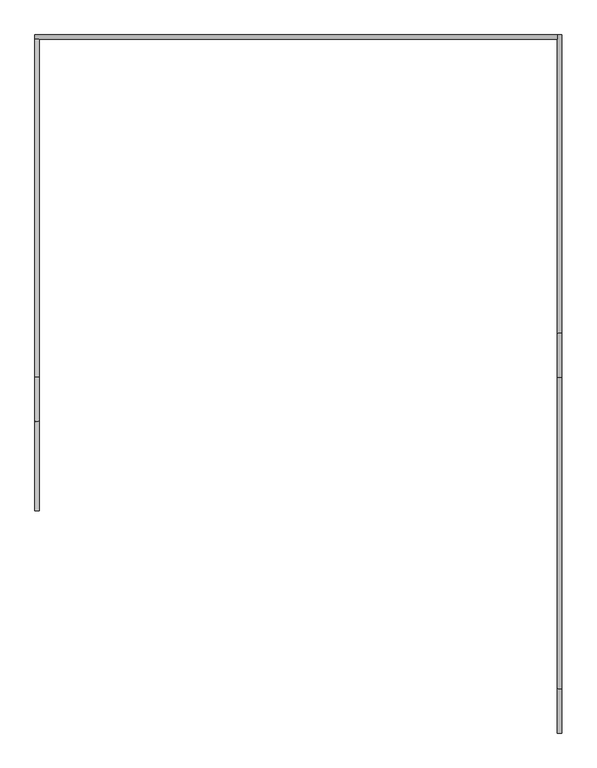
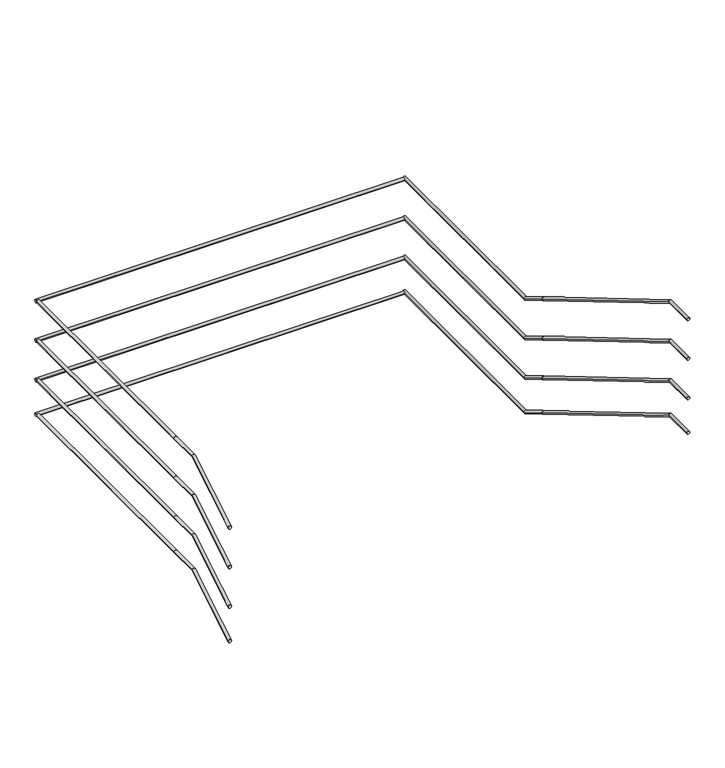
"""IFC4 building model written with IfcOpenShell, lengths in millimetres: railing geometry."""

from ifc_helpers import new_model, si_unit, frame, origin, place, context, project, spatial, circle_curve, ellipse_curve, source, transform, mapped, element, save
from ifc_brep_helpers import plane_surface, cylinder_surface, advanced_brep


def railing_758a8bb7(model_context):
    return source(origin(), model_context, "Body", "AdvancedBrep", [
        advanced_brep(
        [(51115.4, 14329.5208589, 10810.697424), (51085.4, 14329.5208589, 10810.697424), (51115.4, 14933.6395577, 11169.5073179), (51085.4, 14933.6395577, 11169.5073179), (51115.4, 15229.5208589, 11169.5073179), (51085.4, 15229.5208589, 11169.5073179)],
        [
            (0, 1, ellipse_curve(frame((51100.4, 14329.5208589, 10810.697424), z_axis=(0.0, -1.0, 0.0), x_axis=(0.0, 0.0, -1.0)), 17.4462575, 15.0)),
            (1, 0, ellipse_curve(frame((51100.4, 14329.5208589, 10810.697424), z_axis=(0.0, -1.0, 0.0), x_axis=(0.0, 0.0, -1.0)), 17.4462575, 15.0)),
            (0, 2),
            (2, 3, ellipse_curve(frame((51100.4, 14933.6395577, 11169.5073179), z_axis=(0.0, -0.9643088850075937, -0.26477986006381166), x_axis=(0.0, 0.2647798600638126, -0.9643088850075935)), 15.5551818, 15.0)),
            (3, 1),
            (3, 2, ellipse_curve(frame((51100.4, 14933.6395577, 11169.5073179), z_axis=(0.0, -0.9643088850075937, -0.26477986006381166), x_axis=(0.0, 0.2647798600638126, -0.9643088850075935)), 15.5551818, 15.0)),
            (4, 5, circle_curve(frame((51100.4, 15229.5208589, 11169.5073179), z_axis=(0.0, 1.0, 0.0), x_axis=(-1.0, 0.0, 0.0)), 15.0)),
            (5, 4, circle_curve(frame((51100.4, 15229.5208589, 11169.5073179), z_axis=(0.0, 1.0, 0.0), x_axis=(-1.0, 0.0, 0.0)), 15.0)),
            (2, 4),
            (5, 3),
        ],
        [
            plane_surface(frame((51100.4, 14329.5208589, 10828.1436815), z_axis=(0.0, -1.0, 0.0), x_axis=(0.0, 0.0, 1.0))),
            cylinder_surface(frame((51100.4, 14337.180746, 10815.2469328), z_axis=(0.0, -0.8597832514091767, -0.5106591432612018), x_axis=(-1.0, 0.0, 0.0)), 15.0),
            plane_surface(frame((51100.4, 15229.5208589, 11184.5073179), z_axis=(0.0, 1.0, 0.0), x_axis=(0.0, 0.0, 1.0))),
            cylinder_surface(frame((51100.4, 14929.5208589, 11169.5073179), z_axis=(0.0, -1.0, 0.0), x_axis=(-1.0, 0.0, 0.0)), 15.0),
        ],
        [
            (0, [[1, 2]]),
            (1, [[-1, 3, 4, 5]]),
            (1, [[-2, -5, 6, -3]]),
            (2, [[7, 8]]),
            (3, [[-4, 9, -8, 10]]),
            (3, [[-6, -10, -7, -9]]),
        ],
    ),
        advanced_brep(
        [(51115.4, 15229.5208589, 11169.5073179), (51085.4, 15229.5208589, 11169.5073179), (51115.4, 17509.1208589, 11169.5073179), (51085.4, 17509.1208589, 11169.5073179)],
        [
            (0, 1, circle_curve(frame((51100.4, 15229.5208589, 11169.5073179), z_axis=(0.0, -1.0, 0.0), x_axis=(-1.0, 0.0, 0.0)), 15.0)),
            (1, 0, circle_curve(frame((51100.4, 15229.5208589, 11169.5073179), z_axis=(0.0, -1.0, 0.0), x_axis=(-1.0, 0.0, 0.0)), 15.0)),
            (2, 3, circle_curve(frame((51100.4, 17509.1208589, 11169.5073179), z_axis=(0.0, 1.0, 0.0), x_axis=(-1.0, 0.0, 0.0)), 15.0)),
            (3, 2, circle_curve(frame((51100.4, 17509.1208589, 11169.5073179), z_axis=(0.0, 1.0, 0.0), x_axis=(-1.0, 0.0, 0.0)), 15.0)),
            (0, 2),
            (3, 1),
        ],
        [
            plane_surface(frame((51100.4, 15229.5208589, 11184.5073179), z_axis=(0.0, -1.0, 0.0), x_axis=(0.0, 0.0, 1.0))),
            plane_surface(frame((51100.4, 17509.1208589, 11184.5073179), z_axis=(0.0, 1.0, 0.0), x_axis=(0.0, 0.0, 1.0))),
            cylinder_surface(frame((51100.4, 15229.5208589, 11169.5073179), z_axis=(0.0, -1.0, 0.0), x_axis=(-1.0, 0.0, 0.0)), 15.0),
        ],
        [
            (0, [[1, 2]]),
            (1, [[3, 4]]),
            (2, [[-1, 5, -4, 6]]),
            (2, [[-2, -6, -3, -5]]),
        ],
    ),
        advanced_brep(
        [(51085.4, 17509.1208589, 11169.5073179), (51085.4, 17539.1208589, 11169.5073179), (54609.6, 17509.1208589, 11169.5073179), (54609.6, 17539.1208589, 11169.5073179)],
        [
            (0, 1, circle_curve(frame((51085.4, 17524.1208589, 11169.5073179), z_axis=(-1.0, 0.0, 0.0), x_axis=(0.0, 1.0, 0.0)), 15.0)),
            (1, 0, circle_curve(frame((51085.4, 17524.1208589, 11169.5073179), z_axis=(-1.0, 0.0, 0.0), x_axis=(0.0, 1.0, 0.0)), 15.0)),
            (2, 3, circle_curve(frame((54609.6, 17524.1208589, 11169.5073179), z_axis=(1.0, 0.0, 0.0), x_axis=(0.0, 1.0, 0.0)), 15.0)),
            (3, 2, circle_curve(frame((54609.6, 17524.1208589, 11169.5073179), z_axis=(1.0, 0.0, 0.0), x_axis=(0.0, 1.0, 0.0)), 15.0)),
            (0, 2),
            (3, 1),
        ],
        [
            plane_surface(frame((51085.4, 17524.1208589, 11184.5073179), z_axis=(-1.0, 0.0, 0.0), x_axis=(0.0, 1.0, 0.0))),
            plane_surface(frame((54609.6, 17524.1208589, 11184.5073179), z_axis=(1.0, 0.0, 0.0), x_axis=(0.0, 1.0, 0.0))),
            cylinder_surface(frame((51085.4, 17524.1208589, 11169.5073179), z_axis=(-1.0, 0.0, 0.0), x_axis=(0.0, 1.0, 0.0)), 15.0),
        ],
        [
            (0, [[1, 2]]),
            (1, [[3, 4]]),
            (2, [[-1, 5, -4, 6]]),
            (2, [[-2, -6, -3, -5]]),
        ],
    ),
        advanced_brep(
        [(54609.6, 17539.1208589, 11169.5073179), (54639.6, 17539.1208589, 11169.5073179), (54609.6, 15525.40216, 11169.5073179), (54639.6, 15525.40216, 11169.5073179), (54609.6, 15229.5208589, 11345.2428786), (54639.6, 15229.5208589, 11345.2428786)],
        [
            (0, 1, circle_curve(frame((54624.6, 17539.1208589, 11169.5073179), z_axis=(0.0, 1.0, 0.0), x_axis=(1.0, 0.0, 0.0)), 15.0)),
            (1, 0, circle_curve(frame((54624.6, 17539.1208589, 11169.5073179), z_axis=(0.0, 1.0, 0.0), x_axis=(1.0, 0.0, 0.0)), 15.0)),
            (0, 2),
            (2, 3, ellipse_curve(frame((54624.6, 15525.40216, 11169.5073179), z_axis=(0.0, 0.9643088850075936, -0.26477986006381127), x_axis=(0.0, 0.26477986006381177, 0.9643088850075936)), 15.5551818, 15.0)),
            (3, 1),
            (3, 2, ellipse_curve(frame((54624.6, 15525.40216, 11169.5073179), z_axis=(0.0, 0.9643088850075936, -0.26477986006381127), x_axis=(0.0, 0.26477986006381177, 0.9643088850075936)), 15.5551818, 15.0)),
            (4, 5, ellipse_curve(frame((54624.6, 15229.5208589, 11345.2428786), z_axis=(0.0, -1.0, 0.0), x_axis=(0.0, 0.0, -1.0)), 17.4462575, 15.0)),
            (5, 4, ellipse_curve(frame((54624.6, 15229.5208589, 11345.2428786), z_axis=(0.0, -1.0, 0.0), x_axis=(0.0, 0.0, -1.0)), 17.4462575, 15.0)),
            (2, 4),
            (5, 3),
        ],
        [
            plane_surface(frame((54624.6, 17539.1208589, 11184.5073179), z_axis=(0.0, 1.0, 0.0), x_axis=(0.0, 0.0, -1.0))),
            cylinder_surface(frame((54624.6, 17539.1208589, 11169.5073179), z_axis=(0.0, 1.0, 0.0), x_axis=(1.0, 0.0, 0.0)), 15.0),
            plane_surface(frame((54624.6, 15229.5208589, 11362.6891361), z_axis=(0.0, -1.0, 0.0), x_axis=(0.0, 0.0, -1.0))),
            cylinder_surface(frame((54624.6, 15521.8609717, 11171.6105691), z_axis=(0.0, 0.859783251409177, -0.5106591432612011), x_axis=(1.0, 0.0, 0.0)), 15.0),
        ],
        [
            (0, [[1, 2]]),
            (1, [[-1, 3, 4, 5]]),
            (1, [[-2, -5, 6, -3]]),
            (2, [[7, 8]]),
            (3, [[-4, 9, -8, 10]]),
            (3, [[-6, -10, -7, -9]]),
        ],
    ),
        advanced_brep(
        [(54609.6, 15229.5208589, 11345.2428786), (54639.6, 15229.5208589, 11345.2428786), (54609.6, 13125.40216, 12594.9618634), (54639.6, 13125.40216, 12594.9618634), (54609.6, 12829.5208589, 12594.9618634), (54639.6, 12829.5208589, 12594.9618634)],
        [
            (0, 1, ellipse_curve(frame((54624.6, 15229.5208589, 11345.2428786), z_axis=(0.0, 1.0, 0.0), x_axis=(0.0, 0.0, -1.0)), 17.4462575, 15.0)),
            (1, 0, ellipse_curve(frame((54624.6, 15229.5208589, 11345.2428786), z_axis=(0.0, 1.0, 0.0), x_axis=(0.0, 0.0, -1.0)), 17.4462575, 15.0)),
            (0, 2),
            (2, 3, ellipse_curve(frame((54624.6, 13125.40216, 12594.9618634), z_axis=(0.0, 0.9643088850075937, -0.26477986006381166), x_axis=(0.0, -0.2647798600638126, -0.9643088850075935)), 15.5551818, 15.0)),
            (3, 1),
            (3, 2, ellipse_curve(frame((54624.6, 13125.40216, 12594.9618634), z_axis=(0.0, 0.9643088850075937, -0.26477986006381166), x_axis=(0.0, -0.2647798600638126, -0.9643088850075935)), 15.5551818, 15.0)),
            (4, 5, circle_curve(frame((54624.6, 12829.5208589, 12594.9618634), z_axis=(0.0, -1.0, 0.0), x_axis=(1.0, 0.0, 0.0)), 15.0)),
            (5, 4, circle_curve(frame((54624.6, 12829.5208589, 12594.9618634), z_axis=(0.0, -1.0, 0.0), x_axis=(1.0, 0.0, 0.0)), 15.0)),
            (2, 4),
            (5, 3),
        ],
        [
            plane_surface(frame((54624.6, 15229.5208589, 11362.6891361), z_axis=(0.0, 1.0, 0.0), x_axis=(0.0, 0.0, -1.0))),
            cylinder_surface(frame((54624.6, 15221.8609717, 11349.7923873), z_axis=(0.0, 0.8597832514091767, -0.5106591432612018), x_axis=(1.0, 0.0, 0.0)), 15.0),
            plane_surface(frame((54624.6, 12829.5208589, 12609.9618634), z_axis=(0.0, -1.0, 0.0), x_axis=(0.0, 0.0, -1.0))),
            cylinder_surface(frame((54624.6, 13129.5208589, 12594.9618634), z_axis=(0.0, 1.0, 0.0), x_axis=(1.0, 0.0, 0.0)), 15.0),
        ],
        [
            (0, [[1, 2]]),
            (1, [[-1, 3, 4, 5]]),
            (1, [[-2, -5, 6, -3]]),
            (2, [[7, 8]]),
            (3, [[-4, 9, -8, 10]]),
            (3, [[-6, -10, -7, -9]]),
        ],
    ),
        advanced_brep(
        [(51115.4, 14329.5208589, 10010.697424), (51085.4, 14329.5208589, 10010.697424), (51115.4, 14933.6395577, 10369.5073179), (51085.4, 14933.6395577, 10369.5073179), (51115.4, 15229.5208589, 10369.5073179), (51085.4, 15229.5208589, 10369.5073179)],
        [
            (0, 1, ellipse_curve(frame((51100.4, 14329.5208589, 10010.697424), z_axis=(0.0, -1.0, 0.0), x_axis=(0.0, 0.0, -1.0)), 17.4462575, 15.0)),
            (1, 0, ellipse_curve(frame((51100.4, 14329.5208589, 10010.697424), z_axis=(0.0, -1.0, 0.0), x_axis=(0.0, 0.0, -1.0)), 17.4462575, 15.0)),
            (0, 2),
            (2, 3, ellipse_curve(frame((51100.4, 14933.6395577, 10369.5073179), z_axis=(0.0, -0.9643088850075937, -0.26477986006381166), x_axis=(0.0, 0.2647798600638126, -0.9643088850075935)), 15.5551818, 15.0)),
            (3, 1),
            (3, 2, ellipse_curve(frame((51100.4, 14933.6395577, 10369.5073179), z_axis=(0.0, -0.9643088850075937, -0.26477986006381166), x_axis=(0.0, 0.2647798600638126, -0.9643088850075935)), 15.5551818, 15.0)),
            (4, 5, circle_curve(frame((51100.4, 15229.5208589, 10369.5073179), z_axis=(0.0, 1.0, 0.0), x_axis=(-1.0, 0.0, 0.0)), 15.0)),
            (5, 4, circle_curve(frame((51100.4, 15229.5208589, 10369.5073179), z_axis=(0.0, 1.0, 0.0), x_axis=(-1.0, 0.0, 0.0)), 15.0)),
            (2, 4),
            (5, 3),
        ],
        [
            plane_surface(frame((51100.4, 14329.5208589, 10028.1436815), z_axis=(0.0, -1.0, 0.0), x_axis=(0.0, 0.0, 1.0))),
            cylinder_surface(frame((51100.4, 14337.180746, 10015.2469328), z_axis=(0.0, -0.8597832514091767, -0.5106591432612018), x_axis=(-1.0, 0.0, 0.0)), 15.0),
            plane_surface(frame((51100.4, 15229.5208589, 10384.5073179), z_axis=(0.0, 1.0, 0.0), x_axis=(0.0, 0.0, 1.0))),
            cylinder_surface(frame((51100.4, 14929.5208589, 10369.5073179), z_axis=(0.0, -1.0, 0.0), x_axis=(-1.0, 0.0, 0.0)), 15.0),
        ],
        [
            (0, [[1, 2]]),
            (1, [[-1, 3, 4, 5]]),
            (1, [[-2, -5, 6, -3]]),
            (2, [[7, 8]]),
            (3, [[-4, 9, -8, 10]]),
            (3, [[-6, -10, -7, -9]]),
        ],
    ),
        advanced_brep(
        [(51115.4, 15229.5208589, 10369.5073179), (51085.4, 15229.5208589, 10369.5073179), (51115.4, 17509.1208589, 10369.5073179), (51085.4, 17509.1208589, 10369.5073179)],
        [
            (0, 1, circle_curve(frame((51100.4, 15229.5208589, 10369.5073179), z_axis=(0.0, -1.0, 0.0), x_axis=(-1.0, 0.0, 0.0)), 15.0)),
            (1, 0, circle_curve(frame((51100.4, 15229.5208589, 10369.5073179), z_axis=(0.0, -1.0, 0.0), x_axis=(-1.0, 0.0, 0.0)), 15.0)),
            (2, 3, circle_curve(frame((51100.4, 17509.1208589, 10369.5073179), z_axis=(0.0, 1.0, 0.0), x_axis=(-1.0, 0.0, 0.0)), 15.0)),
            (3, 2, circle_curve(frame((51100.4, 17509.1208589, 10369.5073179), z_axis=(0.0, 1.0, 0.0), x_axis=(-1.0, 0.0, 0.0)), 15.0)),
            (0, 2),
            (3, 1),
        ],
        [
            plane_surface(frame((51100.4, 15229.5208589, 10384.5073179), z_axis=(0.0, -1.0, 0.0), x_axis=(0.0, 0.0, 1.0))),
            plane_surface(frame((51100.4, 17509.1208589, 10384.5073179), z_axis=(0.0, 1.0, 0.0), x_axis=(0.0, 0.0, 1.0))),
            cylinder_surface(frame((51100.4, 15229.5208589, 10369.5073179), z_axis=(0.0, -1.0, 0.0), x_axis=(-1.0, 0.0, 0.0)), 15.0),
        ],
        [
            (0, [[1, 2]]),
            (1, [[3, 4]]),
            (2, [[-1, 5, -4, 6]]),
            (2, [[-2, -6, -3, -5]]),
        ],
    ),
        advanced_brep(
        [(51085.4, 17509.1208589, 10369.5073179), (51085.4, 17539.1208589, 10369.5073179), (54609.6, 17509.1208589, 10369.5073179), (54609.6, 17539.1208589, 10369.5073179)],
        [
            (0, 1, circle_curve(frame((51085.4, 17524.1208589, 10369.5073179), z_axis=(-1.0, 0.0, 0.0), x_axis=(0.0, 1.0, 0.0)), 15.0)),
            (1, 0, circle_curve(frame((51085.4, 17524.1208589, 10369.5073179), z_axis=(-1.0, 0.0, 0.0), x_axis=(0.0, 1.0, 0.0)), 15.0)),
            (2, 3, circle_curve(frame((54609.6, 17524.1208589, 10369.5073179), z_axis=(1.0, 0.0, 0.0), x_axis=(0.0, 1.0, 0.0)), 15.0)),
            (3, 2, circle_curve(frame((54609.6, 17524.1208589, 10369.5073179), z_axis=(1.0, 0.0, 0.0), x_axis=(0.0, 1.0, 0.0)), 15.0)),
            (0, 2),
            (3, 1),
        ],
        [
            plane_surface(frame((51085.4, 17524.1208589, 10384.5073179), z_axis=(-1.0, 0.0, 0.0), x_axis=(0.0, 1.0, 0.0))),
            plane_surface(frame((54609.6, 17524.1208589, 10384.5073179), z_axis=(1.0, 0.0, 0.0), x_axis=(0.0, 1.0, 0.0))),
            cylinder_surface(frame((51085.4, 17524.1208589, 10369.5073179), z_axis=(-1.0, 0.0, 0.0), x_axis=(0.0, 1.0, 0.0)), 15.0),
        ],
        [
            (0, [[1, 2]]),
            (1, [[3, 4]]),
            (2, [[-1, 5, -4, 6]]),
            (2, [[-2, -6, -3, -5]]),
        ],
    ),
        advanced_brep(
        [(54609.6, 17539.1208589, 10369.5073179), (54639.6, 17539.1208589, 10369.5073179), (54609.6, 15525.40216, 10369.5073179), (54639.6, 15525.40216, 10369.5073179), (54609.6, 15229.5208589, 10545.2428786), (54639.6, 15229.5208589, 10545.2428786)],
        [
            (0, 1, circle_curve(frame((54624.6, 17539.1208589, 10369.5073179), z_axis=(0.0, 1.0, 0.0), x_axis=(1.0, 0.0, 0.0)), 15.0)),
            (1, 0, circle_curve(frame((54624.6, 17539.1208589, 10369.5073179), z_axis=(0.0, 1.0, 0.0), x_axis=(1.0, 0.0, 0.0)), 15.0)),
            (0, 2),
            (2, 3, ellipse_curve(frame((54624.6, 15525.40216, 10369.5073179), z_axis=(0.0, 0.9643088850075936, -0.26477986006381127), x_axis=(0.0, 0.26477986006381177, 0.9643088850075936)), 15.5551818, 15.0)),
            (3, 1),
            (3, 2, ellipse_curve(frame((54624.6, 15525.40216, 10369.5073179), z_axis=(0.0, 0.9643088850075936, -0.26477986006381127), x_axis=(0.0, 0.26477986006381177, 0.9643088850075936)), 15.5551818, 15.0)),
            (4, 5, ellipse_curve(frame((54624.6, 15229.5208589, 10545.2428786), z_axis=(0.0, -1.0, 0.0), x_axis=(0.0, 0.0, -1.0)), 17.4462575, 15.0)),
            (5, 4, ellipse_curve(frame((54624.6, 15229.5208589, 10545.2428786), z_axis=(0.0, -1.0, 0.0), x_axis=(0.0, 0.0, -1.0)), 17.4462575, 15.0)),
            (2, 4),
            (5, 3),
        ],
        [
            plane_surface(frame((54624.6, 17539.1208589, 10384.5073179), z_axis=(0.0, 1.0, 0.0), x_axis=(0.0, 0.0, -1.0))),
            cylinder_surface(frame((54624.6, 17539.1208589, 10369.5073179), z_axis=(0.0, 1.0, 0.0), x_axis=(1.0, 0.0, 0.0)), 15.0),
            plane_surface(frame((54624.6, 15229.5208589, 10562.6891361), z_axis=(0.0, -1.0, 0.0), x_axis=(0.0, 0.0, -1.0))),
            cylinder_surface(frame((54624.6, 15521.8609717, 10371.6105691), z_axis=(0.0, 0.859783251409177, -0.5106591432612011), x_axis=(1.0, 0.0, 0.0)), 15.0),
        ],
        [
            (0, [[1, 2]]),
            (1, [[-1, 3, 4, 5]]),
            (1, [[-2, -5, 6, -3]]),
            (2, [[7, 8]]),
            (3, [[-4, 9, -8, 10]]),
            (3, [[-6, -10, -7, -9]]),
        ],
    ),
        advanced_brep(
        [(54609.6, 15229.5208589, 10545.2428786), (54639.6, 15229.5208589, 10545.2428786), (54609.6, 13125.40216, 11794.9618634), (54639.6, 13125.40216, 11794.9618634), (54609.6, 12829.5208589, 11794.9618634), (54639.6, 12829.5208589, 11794.9618634)],
        [
            (0, 1, ellipse_curve(frame((54624.6, 15229.5208589, 10545.2428786), z_axis=(0.0, 1.0, 0.0), x_axis=(0.0, 0.0, -1.0)), 17.4462575, 15.0)),
            (1, 0, ellipse_curve(frame((54624.6, 15229.5208589, 10545.2428786), z_axis=(0.0, 1.0, 0.0), x_axis=(0.0, 0.0, -1.0)), 17.4462575, 15.0)),
            (0, 2),
            (2, 3, ellipse_curve(frame((54624.6, 13125.40216, 11794.9618634), z_axis=(0.0, 0.9643088850075937, -0.26477986006381166), x_axis=(0.0, -0.2647798600638126, -0.9643088850075935)), 15.5551818, 15.0)),
            (3, 1),
            (3, 2, ellipse_curve(frame((54624.6, 13125.40216, 11794.9618634), z_axis=(0.0, 0.9643088850075937, -0.26477986006381166), x_axis=(0.0, -0.2647798600638126, -0.9643088850075935)), 15.5551818, 15.0)),
            (4, 5, circle_curve(frame((54624.6, 12829.5208589, 11794.9618634), z_axis=(0.0, -1.0, 0.0), x_axis=(1.0, 0.0, 0.0)), 15.0)),
            (5, 4, circle_curve(frame((54624.6, 12829.5208589, 11794.9618634), z_axis=(0.0, -1.0, 0.0), x_axis=(1.0, 0.0, 0.0)), 15.0)),
            (2, 4),
            (5, 3),
        ],
        [
            plane_surface(frame((54624.6, 15229.5208589, 10562.6891361), z_axis=(0.0, 1.0, 0.0), x_axis=(0.0, 0.0, -1.0))),
            cylinder_surface(frame((54624.6, 15221.8609717, 10549.7923873), z_axis=(0.0, 0.8597832514091767, -0.5106591432612018), x_axis=(1.0, 0.0, 0.0)), 15.0),
            plane_surface(frame((54624.6, 12829.5208589, 11809.9618634), z_axis=(0.0, -1.0, 0.0), x_axis=(0.0, 0.0, -1.0))),
            cylinder_surface(frame((54624.6, 13129.5208589, 11794.9618634), z_axis=(0.0, 1.0, 0.0), x_axis=(1.0, 0.0, 0.0)), 15.0),
        ],
        [
            (0, [[1, 2]]),
            (1, [[-1, 3, 4, 5]]),
            (1, [[-2, -5, 6, -3]]),
            (2, [[7, 8]]),
            (3, [[-4, 9, -8, 10]]),
            (3, [[-6, -10, -7, -9]]),
        ],
    ),
        advanced_brep(
        [(51115.4, 14329.5208589, 10410.697424), (51085.4, 14329.5208589, 10410.697424), (51115.4, 14933.6395577, 10769.5073179), (51085.4, 14933.6395577, 10769.5073179), (51115.4, 15229.5208589, 10769.5073179), (51085.4, 15229.5208589, 10769.5073179)],
        [
            (0, 1, ellipse_curve(frame((51100.4, 14329.5208589, 10410.697424), z_axis=(0.0, -1.0, 0.0), x_axis=(0.0, 0.0, -1.0)), 17.4462575, 15.0)),
            (1, 0, ellipse_curve(frame((51100.4, 14329.5208589, 10410.697424), z_axis=(0.0, -1.0, 0.0), x_axis=(0.0, 0.0, -1.0)), 17.4462575, 15.0)),
            (0, 2),
            (2, 3, ellipse_curve(frame((51100.4, 14933.6395577, 10769.5073179), z_axis=(0.0, -0.9643088850075937, -0.26477986006381166), x_axis=(0.0, 0.2647798600638126, -0.9643088850075935)), 15.5551818, 15.0)),
            (3, 1),
            (3, 2, ellipse_curve(frame((51100.4, 14933.6395577, 10769.5073179), z_axis=(0.0, -0.9643088850075937, -0.26477986006381166), x_axis=(0.0, 0.2647798600638126, -0.9643088850075935)), 15.5551818, 15.0)),
            (4, 5, circle_curve(frame((51100.4, 15229.5208589, 10769.5073179), z_axis=(0.0, 1.0, 0.0), x_axis=(-1.0, 0.0, 0.0)), 15.0)),
            (5, 4, circle_curve(frame((51100.4, 15229.5208589, 10769.5073179), z_axis=(0.0, 1.0, 0.0), x_axis=(-1.0, 0.0, 0.0)), 15.0)),
            (2, 4),
            (5, 3),
        ],
        [
            plane_surface(frame((51100.4, 14329.5208589, 10428.1436815), z_axis=(0.0, -1.0, 0.0), x_axis=(0.0, 0.0, 1.0))),
            cylinder_surface(frame((51100.4, 14337.180746, 10415.2469328), z_axis=(0.0, -0.8597832514091767, -0.5106591432612018), x_axis=(-1.0, 0.0, 0.0)), 15.0),
            plane_surface(frame((51100.4, 15229.5208589, 10784.5073179), z_axis=(0.0, 1.0, 0.0), x_axis=(0.0, 0.0, 1.0))),
            cylinder_surface(frame((51100.4, 14929.5208589, 10769.5073179), z_axis=(0.0, -1.0, 0.0), x_axis=(-1.0, 0.0, 0.0)), 15.0),
        ],
        [
            (0, [[1, 2]]),
            (1, [[-1, 3, 4, 5]]),
            (1, [[-2, -5, 6, -3]]),
            (2, [[7, 8]]),
            (3, [[-4, 9, -8, 10]]),
            (3, [[-6, -10, -7, -9]]),
        ],
    ),
        advanced_brep(
        [(51115.4, 15229.5208589, 10769.5073179), (51085.4, 15229.5208589, 10769.5073179), (51115.4, 17509.1208589, 10769.5073179), (51085.4, 17509.1208589, 10769.5073179)],
        [
            (0, 1, circle_curve(frame((51100.4, 15229.5208589, 10769.5073179), z_axis=(0.0, -1.0, 0.0), x_axis=(-1.0, 0.0, 0.0)), 15.0)),
            (1, 0, circle_curve(frame((51100.4, 15229.5208589, 10769.5073179), z_axis=(0.0, -1.0, 0.0), x_axis=(-1.0, 0.0, 0.0)), 15.0)),
            (2, 3, circle_curve(frame((51100.4, 17509.1208589, 10769.5073179), z_axis=(0.0, 1.0, 0.0), x_axis=(-1.0, 0.0, 0.0)), 15.0)),
            (3, 2, circle_curve(frame((51100.4, 17509.1208589, 10769.5073179), z_axis=(0.0, 1.0, 0.0), x_axis=(-1.0, 0.0, 0.0)), 15.0)),
            (0, 2),
            (3, 1),
        ],
        [
            plane_surface(frame((51100.4, 15229.5208589, 10784.5073179), z_axis=(0.0, -1.0, 0.0), x_axis=(0.0, 0.0, 1.0))),
            plane_surface(frame((51100.4, 17509.1208589, 10784.5073179), z_axis=(0.0, 1.0, 0.0), x_axis=(0.0, 0.0, 1.0))),
            cylinder_surface(frame((51100.4, 15229.5208589, 10769.5073179), z_axis=(0.0, -1.0, 0.0), x_axis=(-1.0, 0.0, 0.0)), 15.0),
        ],
        [
            (0, [[1, 2]]),
            (1, [[3, 4]]),
            (2, [[-1, 5, -4, 6]]),
            (2, [[-2, -6, -3, -5]]),
        ],
    ),
        advanced_brep(
        [(51085.4, 17509.1208589, 10769.5073179), (51085.4, 17539.1208589, 10769.5073179), (54609.6, 17509.1208589, 10769.5073179), (54609.6, 17539.1208589, 10769.5073179)],
        [
            (0, 1, circle_curve(frame((51085.4, 17524.1208589, 10769.5073179), z_axis=(-1.0, 0.0, 0.0), x_axis=(0.0, 1.0, 0.0)), 15.0)),
            (1, 0, circle_curve(frame((51085.4, 17524.1208589, 10769.5073179), z_axis=(-1.0, 0.0, 0.0), x_axis=(0.0, 1.0, 0.0)), 15.0)),
            (2, 3, circle_curve(frame((54609.6, 17524.1208589, 10769.5073179), z_axis=(1.0, 0.0, 0.0), x_axis=(0.0, 1.0, 0.0)), 15.0)),
            (3, 2, circle_curve(frame((54609.6, 17524.1208589, 10769.5073179), z_axis=(1.0, 0.0, 0.0), x_axis=(0.0, 1.0, 0.0)), 15.0)),
            (0, 2),
            (3, 1),
        ],
        [
            plane_surface(frame((51085.4, 17524.1208589, 10784.5073179), z_axis=(-1.0, 0.0, 0.0), x_axis=(0.0, 1.0, 0.0))),
            plane_surface(frame((54609.6, 17524.1208589, 10784.5073179), z_axis=(1.0, 0.0, 0.0), x_axis=(0.0, 1.0, 0.0))),
            cylinder_surface(frame((51085.4, 17524.1208589, 10769.5073179), z_axis=(-1.0, 0.0, 0.0), x_axis=(0.0, 1.0, 0.0)), 15.0),
        ],
        [
            (0, [[1, 2]]),
            (1, [[3, 4]]),
            (2, [[-1, 5, -4, 6]]),
            (2, [[-2, -6, -3, -5]]),
        ],
    ),
        advanced_brep(
        [(54609.6, 17539.1208589, 10769.5073179), (54639.6, 17539.1208589, 10769.5073179), (54609.6, 15525.40216, 10769.5073179), (54639.6, 15525.40216, 10769.5073179), (54609.6, 15229.5208589, 10945.2428786), (54639.6, 15229.5208589, 10945.2428786)],
        [
            (0, 1, circle_curve(frame((54624.6, 17539.1208589, 10769.5073179), z_axis=(0.0, 1.0, 0.0), x_axis=(1.0, 0.0, 0.0)), 15.0)),
            (1, 0, circle_curve(frame((54624.6, 17539.1208589, 10769.5073179), z_axis=(0.0, 1.0, 0.0), x_axis=(1.0, 0.0, 0.0)), 15.0)),
            (0, 2),
            (2, 3, ellipse_curve(frame((54624.6, 15525.40216, 10769.5073179), z_axis=(0.0, 0.9643088850075936, -0.26477986006381127), x_axis=(0.0, 0.26477986006381177, 0.9643088850075936)), 15.5551818, 15.0)),
            (3, 1),
            (3, 2, ellipse_curve(frame((54624.6, 15525.40216, 10769.5073179), z_axis=(0.0, 0.9643088850075936, -0.26477986006381127), x_axis=(0.0, 0.26477986006381177, 0.9643088850075936)), 15.5551818, 15.0)),
            (4, 5, ellipse_curve(frame((54624.6, 15229.5208589, 10945.2428786), z_axis=(0.0, -1.0, 0.0), x_axis=(0.0, 0.0, -1.0)), 17.4462575, 15.0)),
            (5, 4, ellipse_curve(frame((54624.6, 15229.5208589, 10945.2428786), z_axis=(0.0, -1.0, 0.0), x_axis=(0.0, 0.0, -1.0)), 17.4462575, 15.0)),
            (2, 4),
            (5, 3),
        ],
        [
            plane_surface(frame((54624.6, 17539.1208589, 10784.5073179), z_axis=(0.0, 1.0, 0.0), x_axis=(0.0, 0.0, -1.0))),
            cylinder_surface(frame((54624.6, 17539.1208589, 10769.5073179), z_axis=(0.0, 1.0, 0.0), x_axis=(1.0, 0.0, 0.0)), 15.0),
            plane_surface(frame((54624.6, 15229.5208589, 10962.6891361), z_axis=(0.0, -1.0, 0.0), x_axis=(0.0, 0.0, -1.0))),
            cylinder_surface(frame((54624.6, 15521.8609717, 10771.6105691), z_axis=(0.0, 0.859783251409177, -0.5106591432612011), x_axis=(1.0, 0.0, 0.0)), 15.0),
        ],
        [
            (0, [[1, 2]]),
            (1, [[-1, 3, 4, 5]]),
            (1, [[-2, -5, 6, -3]]),
            (2, [[7, 8]]),
            (3, [[-4, 9, -8, 10]]),
            (3, [[-6, -10, -7, -9]]),
        ],
    ),
        advanced_brep(
        [(54609.6, 15229.5208589, 10945.2428786), (54639.6, 15229.5208589, 10945.2428786), (54609.6, 13125.40216, 12194.9618634), (54639.6, 13125.40216, 12194.9618634), (54609.6, 12829.5208589, 12194.9618634), (54639.6, 12829.5208589, 12194.9618634)],
        [
            (0, 1, ellipse_curve(frame((54624.6, 15229.5208589, 10945.2428786), z_axis=(0.0, 1.0, 0.0), x_axis=(0.0, 0.0, -1.0)), 17.4462575, 15.0)),
            (1, 0, ellipse_curve(frame((54624.6, 15229.5208589, 10945.2428786), z_axis=(0.0, 1.0, 0.0), x_axis=(0.0, 0.0, -1.0)), 17.4462575, 15.0)),
            (0, 2),
            (2, 3, ellipse_curve(frame((54624.6, 13125.40216, 12194.9618634), z_axis=(0.0, 0.9643088850075937, -0.26477986006381166), x_axis=(0.0, -0.2647798600638126, -0.9643088850075935)), 15.5551818, 15.0)),
            (3, 1),
            (3, 2, ellipse_curve(frame((54624.6, 13125.40216, 12194.9618634), z_axis=(0.0, 0.9643088850075937, -0.26477986006381166), x_axis=(0.0, -0.2647798600638126, -0.9643088850075935)), 15.5551818, 15.0)),
            (4, 5, circle_curve(frame((54624.6, 12829.5208589, 12194.9618634), z_axis=(0.0, -1.0, 0.0), x_axis=(1.0, 0.0, 0.0)), 15.0)),
            (5, 4, circle_curve(frame((54624.6, 12829.5208589, 12194.9618634), z_axis=(0.0, -1.0, 0.0), x_axis=(1.0, 0.0, 0.0)), 15.0)),
            (2, 4),
            (5, 3),
        ],
        [
            plane_surface(frame((54624.6, 15229.5208589, 10962.6891361), z_axis=(0.0, 1.0, 0.0), x_axis=(0.0, 0.0, -1.0))),
            cylinder_surface(frame((54624.6, 15221.8609717, 10949.7923873), z_axis=(0.0, 0.8597832514091767, -0.5106591432612018), x_axis=(1.0, 0.0, 0.0)), 15.0),
            plane_surface(frame((54624.6, 12829.5208589, 12209.9618634), z_axis=(0.0, -1.0, 0.0), x_axis=(0.0, 0.0, -1.0))),
            cylinder_surface(frame((54624.6, 13129.5208589, 12194.9618634), z_axis=(0.0, 1.0, 0.0), x_axis=(1.0, 0.0, 0.0)), 15.0),
        ],
        [
            (0, [[1, 2]]),
            (1, [[-1, 3, 4, 5]]),
            (1, [[-2, -5, 6, -3]]),
            (2, [[7, 8]]),
            (3, [[-4, 9, -8, 10]]),
            (3, [[-6, -10, -7, -9]]),
        ],
    ),
        advanced_brep(
        [(51115.4, 14329.5208589, 9660.697424), (51085.4, 14329.5208589, 9660.697424), (51115.4, 14933.6395577, 10019.5073179), (51085.4, 14933.6395577, 10019.5073179), (51115.4, 15229.5208589, 10019.5073179), (51085.4, 15229.5208589, 10019.5073179)],
        [
            (0, 1, ellipse_curve(frame((51100.4, 14329.5208589, 9660.697424), z_axis=(0.0, -1.0, 0.0), x_axis=(0.0, 0.0, -1.0)), 17.4462575, 15.0)),
            (1, 0, ellipse_curve(frame((51100.4, 14329.5208589, 9660.697424), z_axis=(0.0, -1.0, 0.0), x_axis=(0.0, 0.0, -1.0)), 17.4462575, 15.0)),
            (0, 2),
            (2, 3, ellipse_curve(frame((51100.4, 14933.6395577, 10019.5073179), z_axis=(0.0, -0.9643088850075937, -0.26477986006381166), x_axis=(0.0, 0.2647798600638126, -0.9643088850075935)), 15.5551818, 15.0)),
            (3, 1),
            (3, 2, ellipse_curve(frame((51100.4, 14933.6395577, 10019.5073179), z_axis=(0.0, -0.9643088850075937, -0.26477986006381166), x_axis=(0.0, 0.2647798600638126, -0.9643088850075935)), 15.5551818, 15.0)),
            (4, 5, circle_curve(frame((51100.4, 15229.5208589, 10019.5073179), z_axis=(0.0, 1.0, 0.0), x_axis=(-1.0, 0.0, 0.0)), 15.0)),
            (5, 4, circle_curve(frame((51100.4, 15229.5208589, 10019.5073179), z_axis=(0.0, 1.0, 0.0), x_axis=(-1.0, 0.0, 0.0)), 15.0)),
            (2, 4),
            (5, 3),
        ],
        [
            plane_surface(frame((51100.4, 14329.5208589, 9678.1436815), z_axis=(0.0, -1.0, 0.0), x_axis=(0.0, 0.0, 1.0))),
            cylinder_surface(frame((51100.4, 14337.180746, 9665.2469328), z_axis=(0.0, -0.8597832514091767, -0.5106591432612018), x_axis=(-1.0, 0.0, 0.0)), 15.0),
            plane_surface(frame((51100.4, 15229.5208589, 10034.5073179), z_axis=(0.0, 1.0, 0.0), x_axis=(0.0, 0.0, 1.0))),
            cylinder_surface(frame((51100.4, 14929.5208589, 10019.5073179), z_axis=(0.0, -1.0, 0.0), x_axis=(-1.0, 0.0, 0.0)), 15.0),
        ],
        [
            (0, [[1, 2]]),
            (1, [[-1, 3, 4, 5]]),
            (1, [[-2, -5, 6, -3]]),
            (2, [[7, 8]]),
            (3, [[-4, 9, -8, 10]]),
            (3, [[-6, -10, -7, -9]]),
        ],
    ),
        advanced_brep(
        [(51115.4, 15229.5208589, 10019.5073179), (51085.4, 15229.5208589, 10019.5073179), (51115.4, 17509.1208589, 10019.5073179), (51085.4, 17509.1208589, 10019.5073179)],
        [
            (0, 1, circle_curve(frame((51100.4, 15229.5208589, 10019.5073179), z_axis=(0.0, -1.0, 0.0), x_axis=(-1.0, 0.0, 0.0)), 15.0)),
            (1, 0, circle_curve(frame((51100.4, 15229.5208589, 10019.5073179), z_axis=(0.0, -1.0, 0.0), x_axis=(-1.0, 0.0, 0.0)), 15.0)),
            (2, 3, circle_curve(frame((51100.4, 17509.1208589, 10019.5073179), z_axis=(0.0, 1.0, 0.0), x_axis=(-1.0, 0.0, 0.0)), 15.0)),
            (3, 2, circle_curve(frame((51100.4, 17509.1208589, 10019.5073179), z_axis=(0.0, 1.0, 0.0), x_axis=(-1.0, 0.0, 0.0)), 15.0)),
            (0, 2),
            (3, 1),
        ],
        [
            plane_surface(frame((51100.4, 15229.5208589, 10034.5073179), z_axis=(0.0, -1.0, 0.0), x_axis=(0.0, 0.0, 1.0))),
            plane_surface(frame((51100.4, 17509.1208589, 10034.5073179), z_axis=(0.0, 1.0, 0.0), x_axis=(0.0, 0.0, 1.0))),
            cylinder_surface(frame((51100.4, 15229.5208589, 10019.5073179), z_axis=(0.0, -1.0, 0.0), x_axis=(-1.0, 0.0, 0.0)), 15.0),
        ],
        [
            (0, [[1, 2]]),
            (1, [[3, 4]]),
            (2, [[-1, 5, -4, 6]]),
            (2, [[-2, -6, -3, -5]]),
        ],
    ),
        advanced_brep(
        [(51085.4, 17509.1208589, 10019.5073179), (51085.4, 17539.1208589, 10019.5073179), (54609.6, 17509.1208589, 10019.5073179), (54609.6, 17539.1208589, 10019.5073179)],
        [
            (0, 1, circle_curve(frame((51085.4, 17524.1208589, 10019.5073179), z_axis=(-1.0, 0.0, 0.0), x_axis=(0.0, 1.0, 0.0)), 15.0)),
            (1, 0, circle_curve(frame((51085.4, 17524.1208589, 10019.5073179), z_axis=(-1.0, 0.0, 0.0), x_axis=(0.0, 1.0, 0.0)), 15.0)),
            (2, 3, circle_curve(frame((54609.6, 17524.1208589, 10019.5073179), z_axis=(1.0, 0.0, 0.0), x_axis=(0.0, 1.0, 0.0)), 15.0)),
            (3, 2, circle_curve(frame((54609.6, 17524.1208589, 10019.5073179), z_axis=(1.0, 0.0, 0.0), x_axis=(0.0, 1.0, 0.0)), 15.0)),
            (0, 2),
            (3, 1),
        ],
        [
            plane_surface(frame((51085.4, 17524.1208589, 10034.5073179), z_axis=(-1.0, 0.0, 0.0), x_axis=(0.0, 1.0, 0.0))),
            plane_surface(frame((54609.6, 17524.1208589, 10034.5073179), z_axis=(1.0, 0.0, 0.0), x_axis=(0.0, 1.0, 0.0))),
            cylinder_surface(frame((51085.4, 17524.1208589, 10019.5073179), z_axis=(-1.0, 0.0, 0.0), x_axis=(0.0, 1.0, 0.0)), 15.0),
        ],
        [
            (0, [[1, 2]]),
            (1, [[3, 4]]),
            (2, [[-1, 5, -4, 6]]),
            (2, [[-2, -6, -3, -5]]),
        ],
    ),
        advanced_brep(
        [(54609.6, 17539.1208589, 10019.5073179), (54639.6, 17539.1208589, 10019.5073179), (54609.6, 15525.40216, 10019.5073179), (54639.6, 15525.40216, 10019.5073179), (54609.6, 15229.5208589, 10195.2428786), (54639.6, 15229.5208589, 10195.2428786)],
        [
            (0, 1, circle_curve(frame((54624.6, 17539.1208589, 10019.5073179), z_axis=(0.0, 1.0, 0.0), x_axis=(1.0, 0.0, 0.0)), 15.0)),
            (1, 0, circle_curve(frame((54624.6, 17539.1208589, 10019.5073179), z_axis=(0.0, 1.0, 0.0), x_axis=(1.0, 0.0, 0.0)), 15.0)),
            (0, 2),
            (2, 3, ellipse_curve(frame((54624.6, 15525.40216, 10019.5073179), z_axis=(0.0, 0.9643088850075936, -0.26477986006381127), x_axis=(0.0, 0.26477986006381177, 0.9643088850075936)), 15.5551818, 15.0)),
            (3, 1),
            (3, 2, ellipse_curve(frame((54624.6, 15525.40216, 10019.5073179), z_axis=(0.0, 0.9643088850075936, -0.26477986006381127), x_axis=(0.0, 0.26477986006381177, 0.9643088850075936)), 15.5551818, 15.0)),
            (4, 5, ellipse_curve(frame((54624.6, 15229.5208589, 10195.2428786), z_axis=(0.0, -1.0, 0.0), x_axis=(0.0, 0.0, -1.0)), 17.4462575, 15.0)),
            (5, 4, ellipse_curve(frame((54624.6, 15229.5208589, 10195.2428786), z_axis=(0.0, -1.0, 0.0), x_axis=(0.0, 0.0, -1.0)), 17.4462575, 15.0)),
            (2, 4),
            (5, 3),
        ],
        [
            plane_surface(frame((54624.6, 17539.1208589, 10034.5073179), z_axis=(0.0, 1.0, 0.0), x_axis=(0.0, 0.0, -1.0))),
            cylinder_surface(frame((54624.6, 17539.1208589, 10019.5073179), z_axis=(0.0, 1.0, 0.0), x_axis=(1.0, 0.0, 0.0)), 15.0),
            plane_surface(frame((54624.6, 15229.5208589, 10212.6891361), z_axis=(0.0, -1.0, 0.0), x_axis=(0.0, 0.0, -1.0))),
            cylinder_surface(frame((54624.6, 15521.8609717, 10021.6105691), z_axis=(0.0, 0.859783251409177, -0.5106591432612011), x_axis=(1.0, 0.0, 0.0)), 15.0),
        ],
        [
            (0, [[1, 2]]),
            (1, [[-1, 3, 4, 5]]),
            (1, [[-2, -5, 6, -3]]),
            (2, [[7, 8]]),
            (3, [[-4, 9, -8, 10]]),
            (3, [[-6, -10, -7, -9]]),
        ],
    ),
        advanced_brep(
        [(54609.6, 15229.5208589, 10195.2428786), (54639.6, 15229.5208589, 10195.2428786), (54609.6, 13125.40216, 11444.9618634), (54639.6, 13125.40216, 11444.9618634), (54609.6, 12829.5208589, 11444.9618634), (54639.6, 12829.5208589, 11444.9618634)],
        [
            (0, 1, ellipse_curve(frame((54624.6, 15229.5208589, 10195.2428786), z_axis=(0.0, 1.0, 0.0), x_axis=(0.0, 0.0, -1.0)), 17.4462575, 15.0)),
            (1, 0, ellipse_curve(frame((54624.6, 15229.5208589, 10195.2428786), z_axis=(0.0, 1.0, 0.0), x_axis=(0.0, 0.0, -1.0)), 17.4462575, 15.0)),
            (0, 2),
            (2, 3, ellipse_curve(frame((54624.6, 13125.40216, 11444.9618634), z_axis=(0.0, 0.9643088850075937, -0.26477986006381166), x_axis=(0.0, -0.2647798600638126, -0.9643088850075935)), 15.5551818, 15.0)),
            (3, 1),
            (3, 2, ellipse_curve(frame((54624.6, 13125.40216, 11444.9618634), z_axis=(0.0, 0.9643088850075937, -0.26477986006381166), x_axis=(0.0, -0.2647798600638126, -0.9643088850075935)), 15.5551818, 15.0)),
            (4, 5, circle_curve(frame((54624.6, 12829.5208589, 11444.9618634), z_axis=(0.0, -1.0, 0.0), x_axis=(1.0, 0.0, 0.0)), 15.0)),
            (5, 4, circle_curve(frame((54624.6, 12829.5208589, 11444.9618634), z_axis=(0.0, -1.0, 0.0), x_axis=(1.0, 0.0, 0.0)), 15.0)),
            (2, 4),
            (5, 3),
        ],
        [
            plane_surface(frame((54624.6, 15229.5208589, 10212.6891361), z_axis=(0.0, 1.0, 0.0), x_axis=(0.0, 0.0, -1.0))),
            cylinder_surface(frame((54624.6, 15221.8609717, 10199.7923873), z_axis=(0.0, 0.8597832514091767, -0.5106591432612018), x_axis=(1.0, 0.0, 0.0)), 15.0),
            plane_surface(frame((54624.6, 12829.5208589, 11459.9618634), z_axis=(0.0, -1.0, 0.0), x_axis=(0.0, 0.0, -1.0))),
            cylinder_surface(frame((54624.6, 13129.5208589, 11444.9618634), z_axis=(0.0, 1.0, 0.0), x_axis=(1.0, 0.0, 0.0)), 15.0),
        ],
        [
            (0, [[1, 2]]),
            (1, [[-1, 3, 4, 5]]),
            (1, [[-2, -5, 6, -3]]),
            (2, [[7, 8]]),
            (3, [[-4, 9, -8, 10]]),
            (3, [[-6, -10, -7, -9]]),
        ],
    ),
    ])


if __name__ == "__main__":
    model = new_model("IFC4")
    model_context = context("Model", 3, world=origin())
    ifc_project = project(units=[si_unit("LENGTHUNIT", "METRE", prefix="MILLI")], contexts=[model_context])
    site = spatial("IfcSite", under=ifc_project)
    building = spatial("IfcBuilding", under=site)
    placement = place(None, origin())
    railing_shape = railing_758a8bb7(model_context)
    element("IfcRailing", 1, at=placement, inside=building, context=model_context, shape_type="MappedRepresentation", body=[
        mapped(railing_shape, transform((0.0, 0.0, 0.0), x_axis=(1.0, 0.0, 0.0), y_axis=(0.0, 1.0, 0.0), z_axis=(0.0, 0.0, 1.0))),
    ])
    save(model, "model.ifc")
